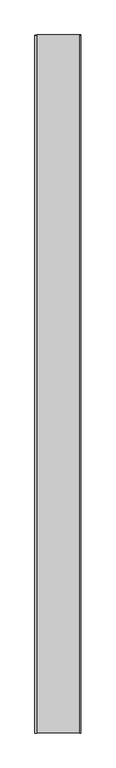
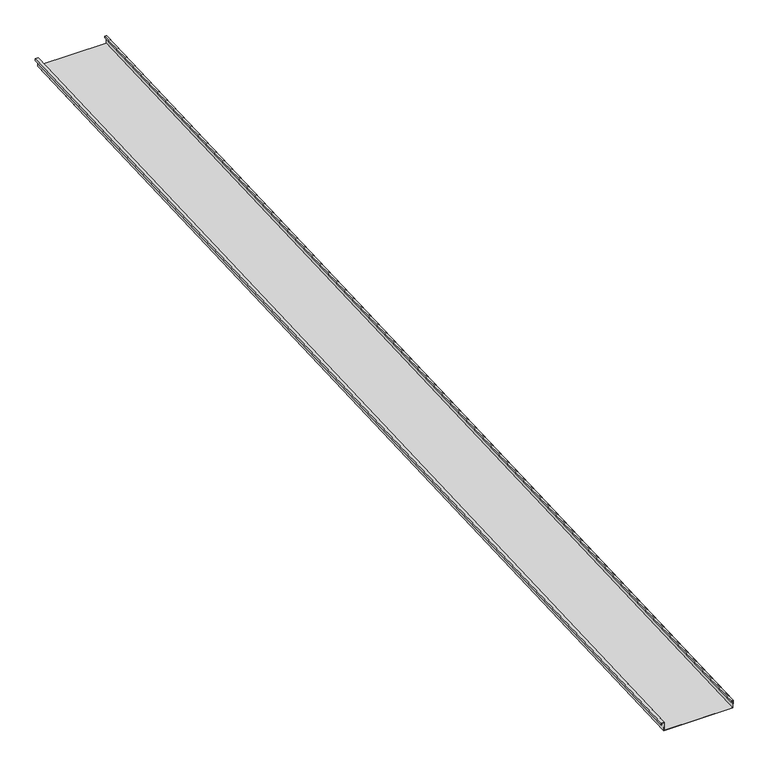
"""IFC4 building model written with IfcOpenShell, lengths in millimetres: proxy geometry, Generic Models 2:Generic Models 2:310765:Generic Models 2:310765 : Generic Models 2:Generic Models 2:310765:102 : Generic Models 2:Generic Models 2:310765:Generic Models 2:310765 : Generic Models 2:Generic Models 2:310765:300385."""

from ifc_helpers import new_model, si_unit, frame, origin, place, context, project, spatial, polyline, outline, extrude, source, transform, mapped, element, save


def generic_models_e11d567a(model_context):
    return source(origin(), model_context, "Body", "SweptSolid", [
        extrude(outline(polyline([(1.5875, 0.0), (1.5875, 50.8), (407.9875, 50.8), (407.9875, 1.5875), (396.875, 1.5875), (396.875, 11.1125), (398.4625, 11.1125), (398.4625, 3.175), (406.4, 3.175), (406.4, 49.2125), (3.175, 49.2125), (3.175, -1.5874999), (-14.2875, -1.5874999), (-14.2875, 9.525), (-12.7, 9.525), (-12.7, 0.0), (1.5875, 0.0)])), frame((613145.0096406, -581354.4345603, 3902.6697972), z_axis=(0.0, 0.9991330730923568, 0.041630544712067834), x_axis=(1.0, 0.0, 0.0)), (0.0, 0.0, 1.0), 6400.8),
    ])


if __name__ == "__main__":
    model = new_model("IFC4")
    model_context = context("Model", 3, world=origin())
    ifc_project = project(units=[si_unit("LENGTHUNIT", "METRE", prefix="MILLI")], contexts=[model_context])
    site = spatial("IfcSite", under=ifc_project)
    building = spatial("IfcBuilding", under=site)
    placement = place(None, origin())
    generic_models_shape = generic_models_e11d567a(model_context)
    element("IfcBuildingElementProxy", 1, Name="Generic Models 2:Generic Models 2:310765:Generic Models 2:310765 : Generic Models 2:Generic Models 2:310765:102 : Generic Models 2:Generic Models 2:310765:Generic Models 2:310765 : Generic Models 2:Generic Models 2:310765:300385", ObjectType="Generic Models 2:Generic Models 2:310765:Generic Models 2:310765 : Generic Models 2:Generic Models 2:310765:102 : Generic Models 2:Generic Models 2:310765:Generic Models 2:310765 : Generic Models 2:Generic Models 2:310765:300385", at=placement, inside=building, context=model_context, shape_type="MappedRepresentation", body=[
        mapped(generic_models_shape, transform((0.0, 0.0, 0.0), x_axis=(1.0, 0.0, 0.0), y_axis=(0.0, 1.0, 0.0), z_axis=(0.0, 0.0, 1.0))),
    ])
    save(model, "model.ifc")

# Revit data of these elements
# Type "Generic Models 2:Generic Models 2:310765:Generic Models 2:310765 : Generic Models 2:Generic Models 2:310765:102 : Generic Models 2:Generic Models 2:310765:Generic Models 2:310765 : Generic Models 2:Generic Models 2:310765:300385"
#   NameOverride = "Generic Models 2:Generic Models 2:310765:Generic Models 2:310765 : Generic Models 2:Generic Models 2:310765:300385"
#   ObjectTypeOverride = "Generic Models 2:310765 : Generic Models 2:Generic Models 2:310765"
#   Reference = "Generic Models 2"
#   Tag = "300385"
# Element 1 (IfcBuildingElementProxy, "Generic Models 2:Generic Models 2:310765:Generic Models 2:310765 : Generic Models 2:Generic Models 2:310765:102 : Generic Models 2:Generic Models 2:310765:Generic Models 2:310765 : Generic Models 2:Generic Models 2:310765:300385")
#   Materials on its faces: "THERMAL BROKEN ALUMINUM STOREFRONT FOR POLYCARBONATE"
# Materials
#   "THERMAL BROKEN ALUMINUM STOREFRONT FOR POLYCARBONATE": class "Unassigned", colour RGB 244 244 244, transparency 0, Keynote = "M07611300.01", Cost = 0
